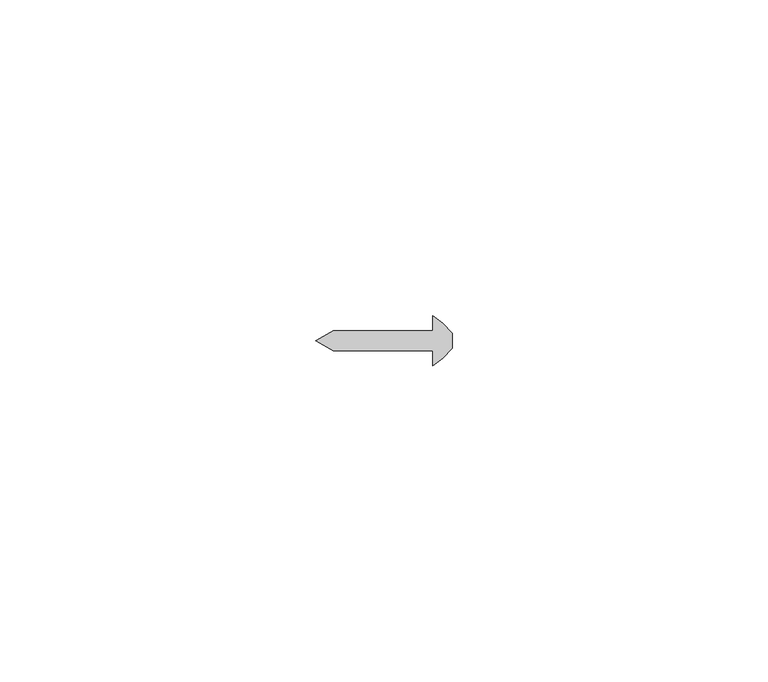
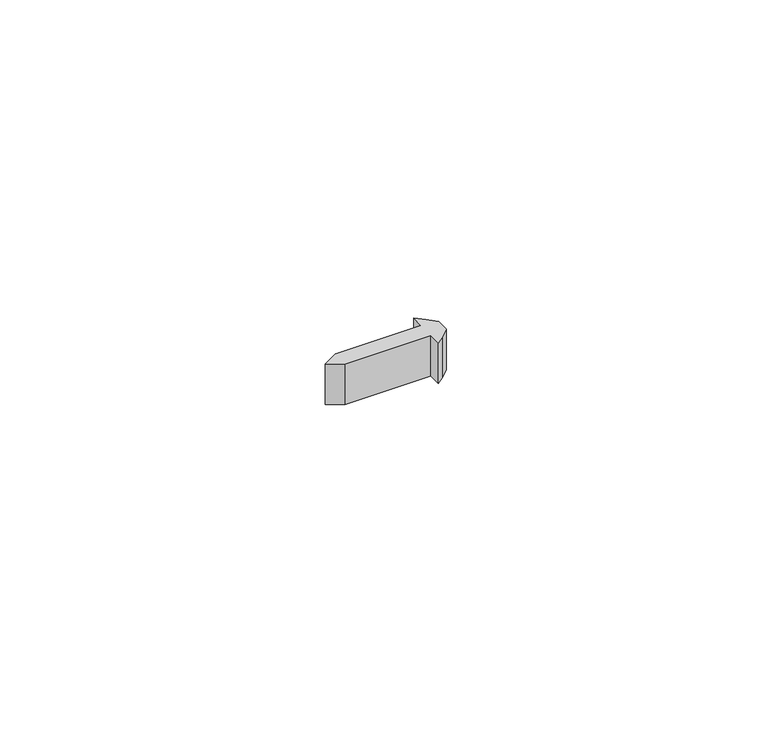
"""IFC4 building model written with IfcOpenShell, lengths in millimetres: proxy geometry, Generic Models 7:Generic Models 1:3:Generic Models 1:3 : Generic Models 7:Generic Models 1:305549:3:Generic Models 1:3:Generic Models 1:3 : Generic Models 7:Generic Models 1:305549:3 : Generic Models 7:Generic Models 1:3:Generic Models 1:3 : Generic Models 7:Generic Models 1:305549:301244:55 : Generic Models 7:Generic Models 1:3:Generic Models 1:3 : Generic Models 7:Generic Models 1:305549:3:Generic Models 1:3:Generic Models 1:3 : Generic Models 7:Generic Models 1:305549:3 : Generic Models 7:Generic Models 1:3:Generic Models 1:3 : Generic Models 7:Generic Models 1:305549:301244:308848."""

from ifc_helpers import new_model, si_unit, frame, origin, place, context, project, spatial, polyline, outline, extrude, source, transform, mapped, element, save


def generic_models_5aac7d62(model_context):
    return source(origin(), model_context, "Body", "SweptSolid", [
        extrude(outline(polyline([(579391.8492239, -578691.1288841), (579391.8492239, -578688.7476341), (579393.3762819, -578689.9658297), (579394.9281721, -578691.5177199), (579394.9281721, -578693.9150483), (579393.3762819, -578695.4669385), (579391.8492239, -578696.6851341), (579391.8492239, -578694.3038841), (579376.0399684, -578694.3038841), (579373.2903377, -578692.7163841), (579376.0399684, -578691.1288841), (579391.8492239, -578691.1288841)])), frame((0.0, 0.0, 4907.75625), z_axis=(0.0, 0.0, 1.0), x_axis=(1.0, 0.0, 0.0)), (0.0, 0.0, 1.0), 7.9375),
    ])


if __name__ == "__main__":
    model = new_model("IFC4")
    model_context = context("Model", 3, world=origin())
    ifc_project = project(units=[si_unit("LENGTHUNIT", "METRE", prefix="MILLI")], contexts=[model_context])
    site = spatial("IfcSite", under=ifc_project)
    building = spatial("IfcBuilding", under=site)
    placement = place(None, origin())
    generic_models_shape = generic_models_5aac7d62(model_context)
    element("IfcBuildingElementProxy", 1, Name="Generic Models 7:Generic Models 1:3:Generic Models 1:3 : Generic Models 7:Generic Models 1:305549:3:Generic Models 1:3:Generic Models 1:3 : Generic Models 7:Generic Models 1:305549:3 : Generic Models 7:Generic Models 1:3:Generic Models 1:3 : Generic Models 7:Generic Models 1:305549:301244:55 : Generic Models 7:Generic Models 1:3:Generic Models 1:3 : Generic Models 7:Generic Models 1:305549:3:Generic Models 1:3:Generic Models 1:3 : Generic Models 7:Generic Models 1:305549:3 : Generic Models 7:Generic Models 1:3:Generic Models 1:3 : Generic Models 7:Generic Models 1:305549:301244:308848", ObjectType="Generic Models 7:Generic Models 1:3:Generic Models 1:3 : Generic Models 7:Generic Models 1:305549:3:Generic Models 1:3:Generic Models 1:3 : Generic Models 7:Generic Models 1:305549:3 : Generic Models 7:Generic Models 1:3:Generic Models 1:3 : Generic Models 7:Generic Models 1:305549:301244:55 : Generic Models 7:Generic Models 1:3:Generic Models 1:3 : Generic Models 7:Generic Models 1:305549:3:Generic Models 1:3:Generic Models 1:3 : Generic Models 7:Generic Models 1:305549:3 : Generic Models 7:Generic Models 1:3:Generic Models 1:3 : Generic Models 7:Generic Models 1:305549:301244:308848", at=placement, inside=building, context=model_context, shape_type="MappedRepresentation", body=[
        mapped(generic_models_shape, transform((0.0, 0.0, 0.0), x_axis=(1.0, 0.0, 0.0), y_axis=(0.0, 1.0, 0.0), z_axis=(0.0, 0.0, 1.0))),
    ])
    save(model, "model.ifc")

# Revit data of these elements
# Type "Generic Models 7:Generic Models 1:3:Generic Models 1:3 : Generic Models 7:Generic Models 1:305549:3:Generic Models 1:3:Generic Models 1:3 : Generic Models 7:Generic Models 1:305549:3 : Generic Models 7:Generic Models 1:3:Generic Models 1:3 : Generic Models 7:Generic Models 1:305549:301244:55 : Generic Models 7:Generic Models 1:3:Generic Models 1:3 : Generic Models 7:Generic Models 1:305549:3:Generic Models 1:3:Generic Models 1:3 : Generic Models 7:Generic Models 1:305549:3 : Generic Models 7:Generic Models 1:3:Generic Models 1:3 : Generic Models 7:Generic Models 1:305549:301244:308848"
#   NameOverride = "Generic Models 7:Generic Models 1:3:Generic Models 1:3 : Generic Models 7:Generic Models 1:305549:3:Generic Models 1:3:Generic Models 1:3 : Generic Models 7:Generic Models 1:305549:3 : Generic Models 7:Generic Models 1:3:Generic Models 1:3 : Generic Models 7:Generic Models 1:305549:301244:308848"
#   ObjectTypeOverride = "Generic Models 1:3:Generic Models 1:3 : Generic Models 7:Generic Models 1:305549:3 : Generic Models 7:Generic Models 1:3:Generic Models 1:3 : Generic Models 7:Generic Models 1:305549:301244"
#   Reference = "Generic Models 1"
#   Tag = "308848"
# Element 1 (IfcBuildingElementProxy, "Generic Models 7:Generic Models 1:3:Generic Models 1:3 : Generic Models 7:Generic Models 1:305549:3:Generic Models 1:3:Generic Models 1:3 : Generic Models 7:Generic Models 1:305549:3 : Generic Models 7:Generic Models 1:3:Generic Models 1:3 : Generic Models 7:Generic Models 1:305549:301244:55 : Generic Models 7:Generic Models 1:3:Generic Models 1:3 : Generic Models 7:Generic Models 1:305549:3:Generic Models 1:3:Generic Models 1:3 : Generic Models 7:Generic Models 1:305549:3 : Generic Models 7:Generic Models 1:3:Generic Models 1:3 : Generic Models 7:Generic Models 1:305549:301244:308848")
#   Materials on its faces: "FASTENERS (T.B.D)"
# Materials
#   "FASTENERS (T.B.D)": class "Generic", colour RGB 120 120 120, transparency 0, Cost = 0
